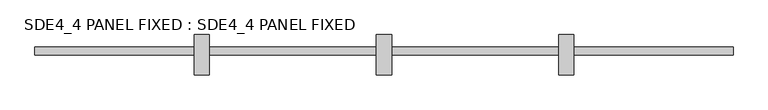
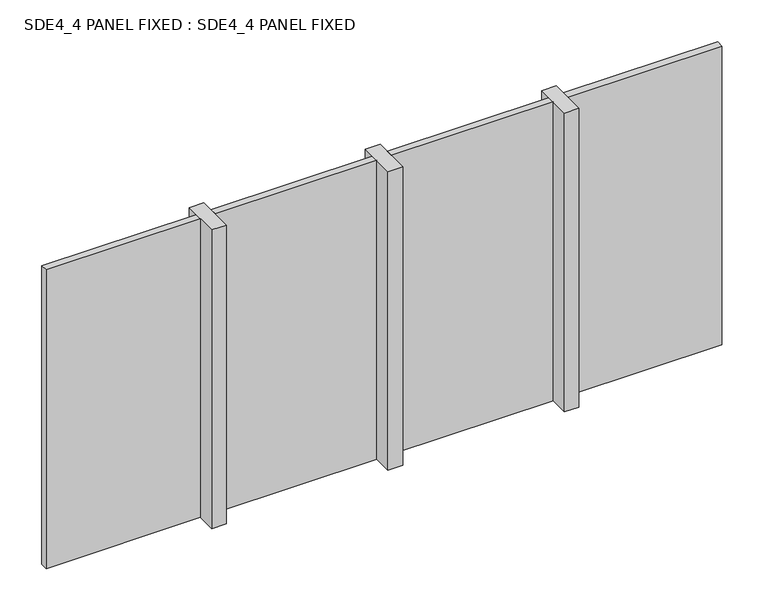
"""IFC4 building model written with IfcOpenShell, lengths in millimetres: plate geometry, SDE4_4 PANEL FIXED : SDE4_4 PANEL FIXED."""

from ifc_helpers import new_model, si_unit, origin, origin_with_axes, place, context, project, spatial, polyline, outline, extrude, source, transform, mapped, element, save


def sde4_4_panel_fixed_sde4_4_panel_fixed_1e2e2a0d(model_context):
    return source(origin(), model_context, "Body", "SweptSolid", [
        extrude(outline(polyline([(-1150.0, 132.5), (-1150.0, -132.5), (-1250.0, -132.5), (-1250.0, 132.5), (-1150.0, 132.5)])), origin_with_axes(), (0.0, 0.0, 1.0), 2149.5956314),
        extrude(outline(polyline([(50.0, 132.5), (50.0, -132.5), (-50.0, -132.5), (-50.0, 132.5), (50.0, 132.5)])), origin_with_axes(), (0.0, 0.0, 1.0), 2149.5956314),
        extrude(outline(polyline([(1250.0, 132.5), (1250.0, -132.5), (1150.0, -132.5), (1150.0, 132.5), (1250.0, 132.5)])), origin_with_axes(), (0.0, 0.0, 1.0), 2149.5956314),
        extrude(outline(polyline([(2299.0, 50.0), (2299.0, 0.0), (1250.0, 0.0), (1250.0, 50.0), (2299.0, 50.0)])), origin_with_axes(), (0.0, 0.0, 1.0), 2149.5956314),
        extrude(outline(polyline([(1150.0, 50.0), (1150.0, 0.0), (50.0, 0.0), (50.0, 50.0), (1150.0, 50.0)])), origin_with_axes(), (0.0, 0.0, 1.0), 2149.5956314),
        extrude(outline(polyline([(-50.0, 50.0), (-50.0, 0.0), (-1150.0, 0.0), (-1150.0, 50.0), (-50.0, 50.0)])), origin_with_axes(), (0.0, 0.0, 1.0), 2149.5956314),
        extrude(outline(polyline([(-1250.0, 50.0), (-1250.0, 0.0), (-2300.0, 0.0), (-2300.0, 50.0), (-1250.0, 50.0)])), origin_with_axes(), (0.0, 0.0, 1.0), 2149.5956314),
    ])


if __name__ == "__main__":
    model = new_model("IFC4")
    model_context = context("Model", 3, world=origin())
    ifc_project = project(units=[si_unit("LENGTHUNIT", "METRE", prefix="MILLI")], contexts=[model_context])
    site = spatial("IfcSite", under=ifc_project)
    building = spatial("IfcBuilding", under=site)
    placement = place(None, origin())
    sde4_4_panel_fixed_sde4_4_panel_fixed_shape = sde4_4_panel_fixed_sde4_4_panel_fixed_1e2e2a0d(model_context)
    element("IfcPlate", 1, ObjectType="SDE4_4 PANEL FIXED : SDE4_4 PANEL FIXED", at=placement, inside=building, context=model_context, shape_type="MappedRepresentation", body=[
        mapped(sde4_4_panel_fixed_sde4_4_panel_fixed_shape, transform((0.0, 0.0, 0.0), x_axis=(1.0, 0.0, 0.0), y_axis=(0.0, 1.0, 0.0), z_axis=(0.0, 0.0, 1.0))),
    ])
    save(model, "model.ifc")

# Revit data of these elements
# Type "SDE4_4 PANEL FIXED : SDE4_4 PANEL FIXED"
#   Type Mark = "CW-GLASS"
#   Analytic Construction = "<None>"
#   Glass = Glass
#   Frame = Aluminium
# Element 1 (IfcPlate, "SDE4_4 PANEL FIXED : SDE4_4 PANEL FIXED")
#   Materials on its faces: "Glass", "Aluminium"
# Materials
#   "Glass": class "Glass", colour RGB 0 128 192, transparency 0.9, Keynote = "L40", Cost = 0
#   "Aluminium": class "Unassigned", colour RGB 247 247 247, transparency 0, Cost = 0
